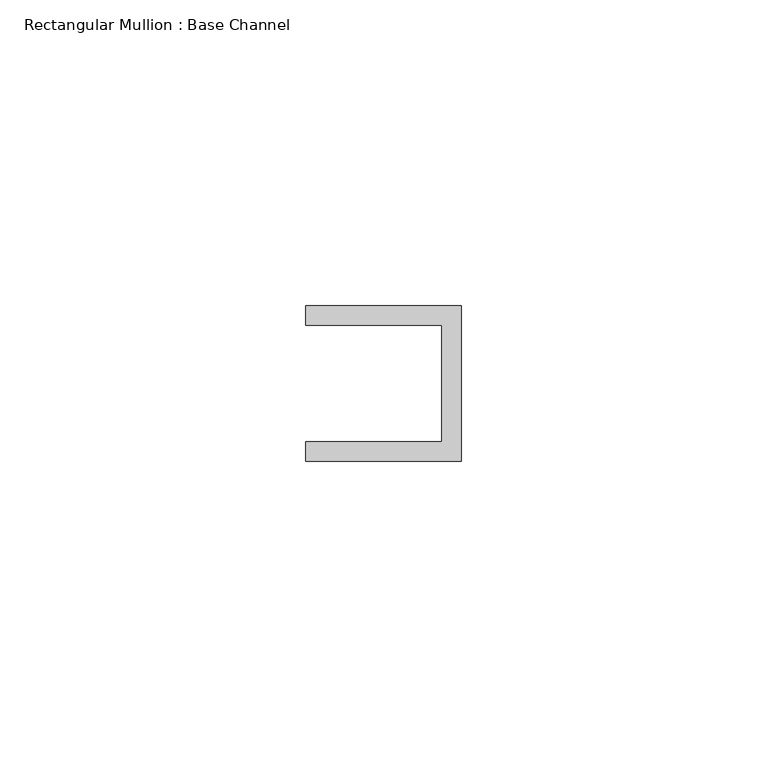
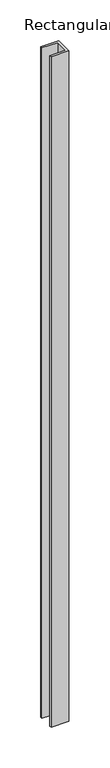
"""IFC4 building model written with IfcOpenShell, lengths in millimetres: member geometry, Rectangular Mullion : Base Channel."""

from ifc_helpers import new_model, si_unit, frame, origin, place, context, project, spatial, polyline, outline, extrude, source, transform, mapped, element, save


def rectangular_mullion_base_channel_45555192(model_context):
    return source(origin(), model_context, "Body", "SweptSolid", [
        extrude(outline(polyline([(0.0, -12.7), (-25.4, -12.7), (-25.4, -9.525), (-3.175, -9.525), (-3.175, 9.525), (-25.4, 9.525), (-25.4, 12.7), (0.0, 12.7), (0.0, -12.7)])), frame((0.0, 0.0, -1005.4166667), z_axis=(0.0, 0.0, 1.0), x_axis=(1.0, 0.0, 0.0)), (0.0, 0.0, 1.0), 1005.4166667),
    ])


if __name__ == "__main__":
    model = new_model("IFC4")
    model_context = context("Model", 3, world=origin())
    ifc_project = project(units=[si_unit("LENGTHUNIT", "METRE", prefix="MILLI")], contexts=[model_context])
    site = spatial("IfcSite", under=ifc_project)
    building = spatial("IfcBuilding", under=site)
    placement = place(None, origin())
    rectangular_mullion_base_channel_shape = rectangular_mullion_base_channel_45555192(model_context)
    element("IfcMember", 1, ObjectType="Rectangular Mullion : Base Channel", at=placement, inside=building, context=model_context, shape_type="MappedRepresentation", body=[
        mapped(rectangular_mullion_base_channel_shape, transform((0.0, 0.0, 0.0), x_axis=(1.0, 0.0, 0.0), y_axis=(0.0, 1.0, 0.0), z_axis=(0.0, 0.0, 1.0))),
    ])
    save(model, "model.ifc")

# Revit data of these elements
# Type "Rectangular Mullion : Base Channel"
#   built-in parameter 1007322 = 0.0833333 (stored number, unit not read)
#   built-in parameter 1007321 = 0.0416667 (stored number, unit not read)
#   built-in parameter 1007320 = -0.03125 (stored number, unit not read)
# Element 1 (IfcMember, "Rectangular Mullion : Base Channel")
#   Materials on its faces: "ALUM"
# Materials
#   "ALUM": class "Generic", colour RGB 157 157 157, transparency 0, Cost = 0
